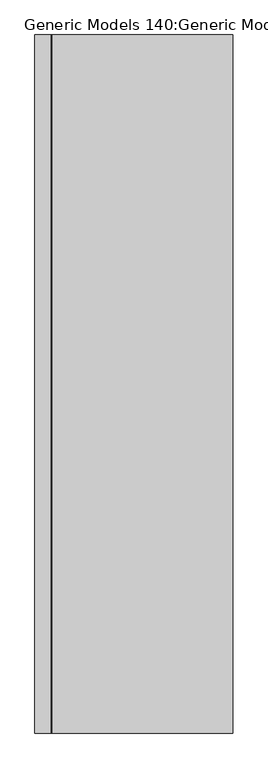
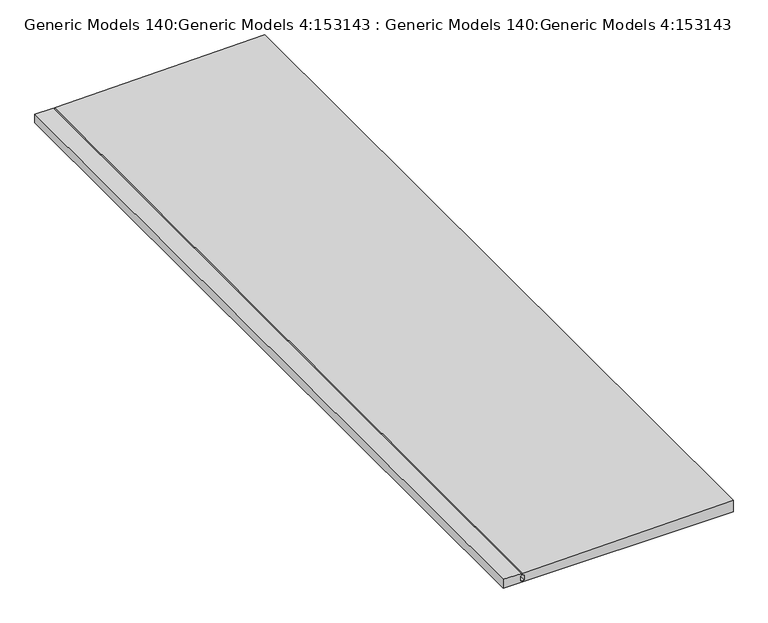
"""IFC4 building model written with IfcOpenShell, lengths in millimetres: proxy geometry, Generic Models 140:Generic Models 4:153143 : Generic Models 140:Generic Models 4:153143."""

from ifc_helpers import new_model, si_unit, frame, origin, place, context, project, spatial, polyline, outline, extrude, source, transform, mapped, element, save


def generic_models_140_generic_models_4_153143_generic_models_684afeb2(model_context):
    return source(origin(), model_context, "Body", "SweptSolid", [
        extrude(outline(polyline([(-199.6449764, -10331.3078813), (-342.0475126, -10331.3078813), (-342.0475126, -6772.396787), (-147.8591793, -6772.396787), (-204.6132116, -10023.8331192), (-234.8858169, -10023.8331192), (-244.697406, -10005.4599184), (-319.9504847, -10005.4599184), (-333.2189606, -10036.0328813), (-318.3595518, -10065.7849184), (-243.0709843, -10065.7849184), (-234.778648, -10046.6778792), (-204.6132116, -10046.6778792), (-199.6449764, -10331.3078813)])), frame((0.0, -5303.1974793, 0.0), z_axis=(0.0, 1.0, 0.0), x_axis=(0.0, 0.0, 1.0)), (0.0, 0.0, 1.0), 12547.6),
    ])


if __name__ == "__main__":
    model = new_model("IFC4")
    model_context = context("Model", 3, world=origin())
    ifc_project = project(units=[si_unit("LENGTHUNIT", "METRE", prefix="MILLI")], contexts=[model_context])
    site = spatial("IfcSite", under=ifc_project)
    building = spatial("IfcBuilding", under=site)
    placement = place(None, origin())
    generic_models_140_generic_models_4_153143_generic_models_shape = generic_models_140_generic_models_4_153143_generic_models_684afeb2(model_context)
    element("IfcBuildingElementProxy", 1, Name="Generic Models 140:Generic Models 4:153143 : Generic Models 140:Generic Models 4:153143", ObjectType="Generic Models 140:Generic Models 4:153143 : Generic Models 140:Generic Models 4:153143", at=placement, inside=building, context=model_context, shape_type="MappedRepresentation", body=[
        mapped(generic_models_140_generic_models_4_153143_generic_models_shape, transform((0.0, 0.0, 0.0), x_axis=(1.0, 0.0, 0.0), y_axis=(0.0, 1.0, 0.0), z_axis=(0.0, 0.0, 1.0))),
    ])
    save(model, "model.ifc")

# Revit data of these elements
# Type "Generic Models 140:Generic Models 4:153143 : Generic Models 140:Generic Models 4:153143"
#   NameOverride = "Generic Models 140:Generic Models 4:153143"
#   ObjectTypeOverride = "Generic Models 140:Generic Models 4"
#   Reference = "Generic Models 4"
#   Category = "Generic Models"
#   Tag = "153143"
# Element 1 (IfcBuildingElementProxy, "Generic Models 140:Generic Models 4:153143 : Generic Models 140:Generic Models 4:153143")
#   Materials on its faces: "_CONCRETE SLAB W/ WIRE MESH (SEE STRUCT. DWGS) - SLOPE 1% AWAY FROM BUILDING 9884"
# Materials
#   "_CONCRETE SLAB W/ WIRE MESH (SEE STRUCT. DWGS) - SLOPE 1% AWAY FROM BUILDING 9884": class "Unassigned", colour RGB 191 191 191, transparency 0
